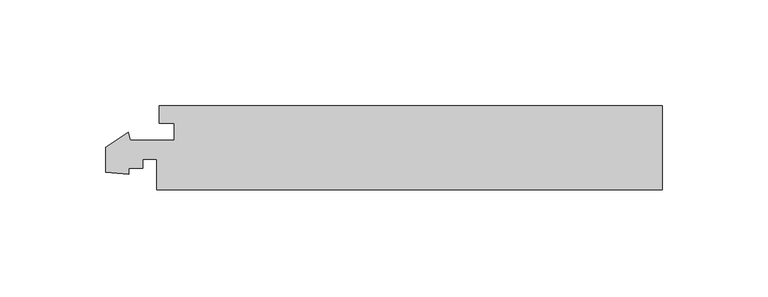
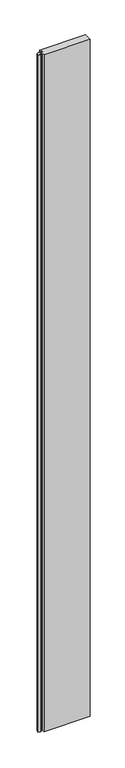
"""IFC4 building model written with IfcOpenShell, lengths in millimetres: proxy geometry, Generic Models 5:Generic Models 5:321804:Generic Models 5:321804 : Generic Models 5:Generic Models 5:321804:28 : Generic Models 5:Generic Models 5:321804:Generic Models 5:321804 : Generic Models 5:Generic Models 5:321804:300761."""

from ifc_helpers import new_model, si_unit, frame, origin, place, context, project, spatial, polyline, outline, extrude, source, transform, mapped, element, save


def generic_models_146d81d0(model_context):
    return source(origin(), model_context, "Body", "SweptSolid", [
        extrude(outline(polyline([(667278.0673246, -568197.4413841), (667516.4165209, -568197.4413841), (667516.4165209, -568237.4413841), (667276.8173246, -568237.4413841), (667276.8173246, -568222.9413841), (667270.1923246, -568222.9413841), (667270.1923246, -568227.2413841), (667263.5673246, -568227.2413841), (667263.5673246, -568229.9413841), (667252.5673246, -568228.9790088), (667252.5673246, -568217.1208678), (667263.2488265, -568210.0135026), (667264.3012992, -568213.9413841), (667285.0173246, -568213.9413841), (667285.0173246, -568205.9413841), (667278.0673246, -568205.9413841), (667278.0673246, -568197.4413841)])), frame((0.0, 0.0, 6217.7309013), z_axis=(0.0, 0.0, 1.0), x_axis=(1.0, 0.0, 0.0)), (0.0, 0.0, 1.0), 3701.5636234),
    ])


if __name__ == "__main__":
    model = new_model("IFC4")
    model_context = context("Model", 3, world=origin())
    ifc_project = project(units=[si_unit("LENGTHUNIT", "METRE", prefix="MILLI")], contexts=[model_context])
    site = spatial("IfcSite", under=ifc_project)
    building = spatial("IfcBuilding", under=site)
    placement = place(None, origin())
    generic_models_shape = generic_models_146d81d0(model_context)
    element("IfcBuildingElementProxy", 1, Name="Generic Models 5:Generic Models 5:321804:Generic Models 5:321804 : Generic Models 5:Generic Models 5:321804:28 : Generic Models 5:Generic Models 5:321804:Generic Models 5:321804 : Generic Models 5:Generic Models 5:321804:300761", ObjectType="Generic Models 5:Generic Models 5:321804:Generic Models 5:321804 : Generic Models 5:Generic Models 5:321804:28 : Generic Models 5:Generic Models 5:321804:Generic Models 5:321804 : Generic Models 5:Generic Models 5:321804:300761", at=placement, inside=building, context=model_context, shape_type="MappedRepresentation", body=[
        mapped(generic_models_shape, transform((0.0, 0.0, 0.0), x_axis=(1.0, 0.0, 0.0), y_axis=(0.0, 1.0, 0.0), z_axis=(0.0, 0.0, 1.0))),
    ])
    save(model, "model.ifc")

# Revit data of these elements
# Type "Generic Models 5:Generic Models 5:321804:Generic Models 5:321804 : Generic Models 5:Generic Models 5:321804:28 : Generic Models 5:Generic Models 5:321804:Generic Models 5:321804 : Generic Models 5:Generic Models 5:321804:300761"
#   NameOverride = "Generic Models 5:Generic Models 5:321804:Generic Models 5:321804 : Generic Models 5:Generic Models 5:321804:300761"
#   ObjectTypeOverride = "Generic Models 5:321804 : Generic Models 5:Generic Models 5:321804"
#   Reference = "Generic Models 5"
#   Tag = "300761"
# Element 1 (IfcBuildingElementProxy, "Generic Models 5:Generic Models 5:321804:Generic Models 5:321804 : Generic Models 5:Generic Models 5:321804:28 : Generic Models 5:Generic Models 5:321804:Generic Models 5:321804 : Generic Models 5:Generic Models 5:321804:300761")
#   Materials on its faces: "POLYCARBONATE PANEL - ARCOPLUS 547"
# Materials
#   "POLYCARBONATE PANEL - ARCOPLUS 547": class "Unassigned", colour RGB 202 225 249, transparency 0.45, Cost = 0
